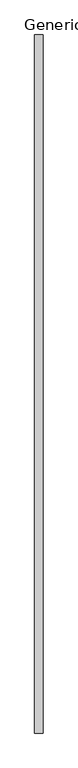
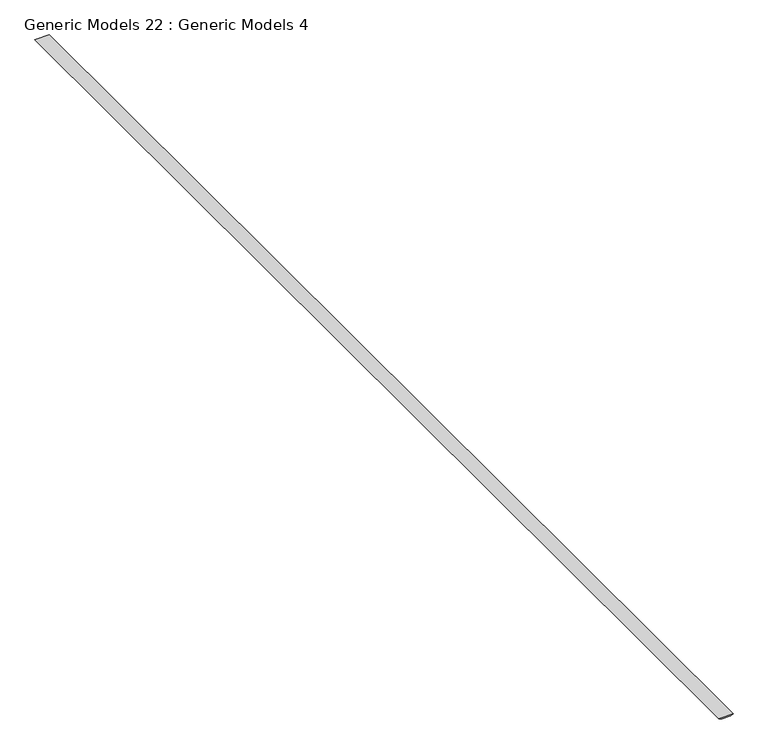
"""IFC4 building model written with IfcOpenShell, lengths in millimetres: proxy geometry, Generic Models 22 : Generic Models 4."""

from ifc_helpers import new_model, si_unit, frame, origin, place, context, project, spatial, polyline, outline, extrude, source, transform, mapped, element, save


def generic_models_22_generic_models_4_f07917f7(model_context):
    return source(origin(), model_context, "Body", "SweptSolid", [
        extrude(outline(polyline([(127085.980596, 8404.419308), (127089.1652967, 8559.799908), (127107.6883511, 8595.8711192), (127103.0817625, 8371.1170363), (127085.980596, 8404.419308)])), frame((0.0, -6864.9230338, 0.0), z_axis=(0.0, 1.0, 0.0), x_axis=(0.0, 0.0, 1.0)), (0.0, 0.0, 1.0), 18643.6),
    ])


if __name__ == "__main__":
    model = new_model("IFC4")
    model_context = context("Model", 3, world=origin())
    ifc_project = project(units=[si_unit("LENGTHUNIT", "METRE", prefix="MILLI")], contexts=[model_context])
    site = spatial("IfcSite", under=ifc_project)
    building = spatial("IfcBuilding", under=site)
    placement = place(None, origin())
    generic_models_22_generic_models_4_shape = generic_models_22_generic_models_4_f07917f7(model_context)
    element("IfcBuildingElementProxy", 1, Name="Generic Models 22 : Generic Models 4", ObjectType="Generic Models 22 : Generic Models 4", at=placement, inside=building, context=model_context, shape_type="MappedRepresentation", body=[
        mapped(generic_models_22_generic_models_4_shape, transform((0.0, 0.0, 0.0), x_axis=(1.0, 0.0, 0.0), y_axis=(0.0, 1.0, 0.0), z_axis=(0.0, 0.0, 1.0))),
    ])
    save(model, "model.ifc")

# Revit data of these elements
# Element 1 (IfcBuildingElementProxy, "Generic Models 22 : Generic Models 4")
#   Materials on its faces: "_7/8\" SMOOTH TROWEL EXTERIOR STUCCO (COLOR PER OWNER) @ 2% SLOPE"
# Materials
#   "_7/8\" SMOOTH TROWEL EXTERIOR STUCCO (COLOR PER OWNER) @ 2% SLOPE": class "Generic", colour RGB 233 233 233, transparency 0, Cost = 0
